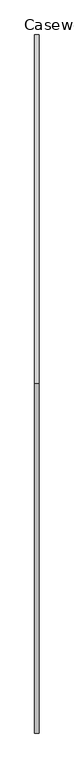
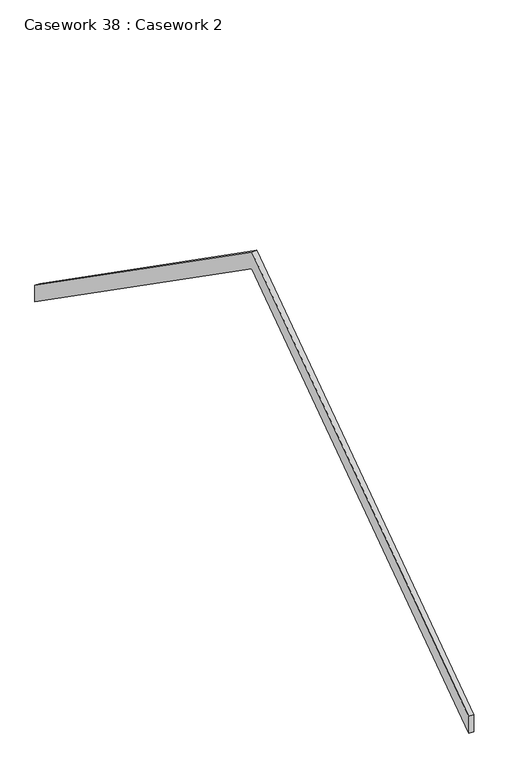
"""IFC4 building model written with IfcOpenShell, lengths in millimetres: furniture geometry, Casework 38 : Casework 2."""

import ifcopenshell
import ifcopenshell.guid

model = None  # the IFC model being written
_history = None  # IfcOwnerHistory: only IFC2X3 demands one
_inside = {}  # id of a spatial element -> (the spatial element, [elements in it])
_under = {}  # id of a project, library or spatial element -> (it, [spatial elements below it])
_declared = {}  # id of a project -> (the project, [libraries it declares])
_typed = {}  # id of a type object -> (the type object, [elements of that type])
_made_of = {}  # id of a material, layer set ... -> (it, [elements and type objects made of it])


def new_model(schema):
    """Start an empty IFC model of exactly this schema.

    Asked for "IFC4X3", IfcOpenShell would pick the latest addendum, in which some entities
    have other attributes; the version numbers below select the first issue.
    IFC2X3 requires an IfcOwnerHistory on every rooted entity: one is made here for all.
    """
    global model, _history
    if schema == "IFC4X3":
        model = ifcopenshell.file(schema_version=(4, 3, 0, 0))
    else:
        model = ifcopenshell.file(schema=schema)
    _inside.clear()
    _under.clear()
    _declared.clear()
    _typed.clear()
    _made_of.clear()
    _history = None
    if model.schema == "IFC2X3":
        org = make("IfcOrganization", Name="unknown")
        user = make(
            "IfcPersonAndOrganization",
            ThePerson=make("IfcPerson", FamilyName="unknown"),
            TheOrganization=org,
        )
        app = make(
            "IfcApplication",
            ApplicationDeveloper=org,
            Version="unknown",
            ApplicationFullName="unknown",
            ApplicationIdentifier="unknown",
        )
        _history = make(
            "IfcOwnerHistory",
            OwningUser=user,
            OwningApplication=app,
            ChangeAction="ADDED",
            CreationDate=0,
        )
    return model


def make(cls, **values):
    """One entity of the class cls with the attributes given. An attribute that is None is left unset."""
    return model.create_entity(
        cls, **{name: value for name, value in values.items() if value is not None}
    )


def rooted(cls, **values):
    """An entity with a GlobalId (a new one), such as an element, a storey or a relation."""
    return make(cls, GlobalId=ifcopenshell.guid.new(), OwnerHistory=_history, **values)


def si_unit(unit_type, name, prefix=None):
    """IfcSIUnit, for example si_unit("LENGTHUNIT", "METRE", prefix="MILLI")."""
    return make("IfcSIUnit", UnitType=unit_type, Prefix=prefix, Name=name)


def assignment(units):
    """IfcUnitAssignment: the units of a project."""
    return None if units is None else make("IfcUnitAssignment", Units=units)


def point(xyz):
    """IfcCartesianPoint."""
    return None if xyz is None else make("IfcCartesianPoint", Coordinates=xyz)


def direction(xyz):
    """IfcDirection."""
    return None if xyz is None else make("IfcDirection", DirectionRatios=xyz)


def frame(location, z_axis=None, x_axis=None):
    """IfcAxis2Placement3D, a coordinate frame: its origin and axes. An axis left out is left unset."""
    return make(
        "IfcAxis2Placement3D",
        Location=point(location),
        Axis=direction(z_axis),
        RefDirection=direction(x_axis),
    )


def origin():
    """The frame at (0, 0, 0) with its axes left unset."""
    return frame((0.0, 0.0, 0.0))


def place(relative_to, where):
    """IfcLocalPlacement: puts the frame where relative to a parent placement (None: the world)."""
    return make(
        "IfcLocalPlacement", PlacementRelTo=relative_to, RelativePlacement=where
    )


def context(
    kind, dimensions, precision=None, world=None, true_north=None, identifier=None
):
    """IfcGeometricRepresentationContext, for example the 3D "Model" context."""
    return make(
        "IfcGeometricRepresentationContext",
        ContextIdentifier=identifier,
        ContextType=kind,
        CoordinateSpaceDimension=dimensions,
        Precision=precision,
        WorldCoordinateSystem=world,
        TrueNorth=true_north,
    )


def project(units=None, contexts=None):
    """IfcProject with its units and contexts."""
    return rooted(
        "IfcProject",
        Name="project",
        RepresentationContexts=contexts,
        UnitsInContext=assignment(units),
    )


def spatial(cls, under=None, at=None, **own):
    """A site, building, storey or space (cls), placed at a placement, below another one or the project."""
    s = rooted(cls, ObjectPlacement=at, **own)
    if under is not None:
        _under.setdefault(under.id(), (under, []))[1].append(s)
    return s


def polyline(points):
    """IfcPolyline through the points."""
    return make("IfcPolyline", Points=[point(p) for p in points])


def outline(outer, holes=None, kind="AREA"):
    """IfcArbitraryClosedProfileDef: a profile drawn as a closed curve; with holes, ...WithVoids."""
    if holes is None:
        return make("IfcArbitraryClosedProfileDef", ProfileType=kind, OuterCurve=outer)
    return make(
        "IfcArbitraryProfileDefWithVoids",
        ProfileType=kind,
        OuterCurve=outer,
        InnerCurves=holes,
    )


def extrude(swept, where, along, depth):
    """IfcExtrudedAreaSolid: the profile swept, set in the frame where, extruded along a direction by depth."""
    return make(
        "IfcExtrudedAreaSolid",
        SweptArea=swept,
        Position=where,
        ExtrudedDirection=direction(along),
        Depth=depth,
    )


def shape(context_of_items, identifier, shape_type, items):
    """IfcShapeRepresentation: the items that make up one representation, for example the "Body"."""
    return make(
        "IfcShapeRepresentation",
        ContextOfItems=context_of_items,
        RepresentationIdentifier=identifier,
        RepresentationType=shape_type,
        Items=items,
    )


def source(mapping_origin, context_of_items, identifier, shape_type, items):
    """IfcRepresentationMap: a shape defined once, which mapped items show again and again."""
    return make(
        "IfcRepresentationMap",
        MappingOrigin=mapping_origin,
        MappedRepresentation=shape(context_of_items, identifier, shape_type, items),
    )


def transform(
    local_origin,
    x_axis=None,
    y_axis=None,
    z_axis=None,
    scale=None,
    scale2=None,
    scale3=None,
    uniform=True,
):
    """IfcCartesianTransformationOperator3D, or its non-uniform kind. x_axis, y_axis, z_axis: its Axis1, 2, 3."""
    if uniform:
        return make(
            "IfcCartesianTransformationOperator3D",
            Axis1=direction(x_axis),
            Axis2=direction(y_axis),
            LocalOrigin=point(local_origin),
            Scale=scale,
            Axis3=direction(z_axis),
        )
    return make(
        "IfcCartesianTransformationOperator3DnonUniform",
        Axis1=direction(x_axis),
        Axis2=direction(y_axis),
        LocalOrigin=point(local_origin),
        Scale=scale,
        Axis3=direction(z_axis),
        Scale2=scale2,
        Scale3=scale3,
    )


def mapped(mapping_source, mapping_target):
    """IfcMappedItem: shows the shape of a source again, moved by a transform."""
    return make(
        "IfcMappedItem", MappingSource=mapping_source, MappingTarget=mapping_target
    )


def made_of(thing, what):
    """Note that an element or type object is made of a material, layer set ...; save() writes the relation."""
    if what is not None:
        _made_of.setdefault(what.id(), (what, []))[1].append(thing)
    return thing


def element(
    cls,
    number,
    at=None,
    inside=None,
    cuts=None,
    type_object=None,
    material=None,
    context=None,
    identifier="Body",
    shape_type=None,
    held_by="IfcProductDefinitionShape",
    body=None,
    shapes=None,
    **own,
):
    """One element of the class cls, such as IfcWall. Its Tag is "e" and its number.

    at: its placement. inside: the storey or other place that contains it. cuts: it is an
    opening in that element (IfcRelVoidsElement). A single representation is given by context,
    identifier, shape_type and body (its items); several are given by shapes. held_by: the class
    of the entity that holds the representations. save() writes the other relations.
    """
    e = rooted(cls, Tag="e%d" % number, ObjectPlacement=at, **own)
    if body is not None:
        shapes = [shape(context, identifier, shape_type, body)]
    if shapes is not None:
        e.Representation = make(held_by, Representations=shapes)
    if inside is not None:
        _inside.setdefault(inside.id(), (inside, []))[1].append(e)
    if cuts is not None:
        rooted(
            "IfcRelVoidsElement", RelatingBuildingElement=cuts, RelatedOpeningElement=e
        )
    if type_object is not None:
        _typed.setdefault(type_object.id(), (type_object, []))[1].append(e)
    return made_of(e, material)


def aggregate(whole, parts):
    """IfcRelAggregates: a whole, such as a stair, and the parts it consists of."""
    return rooted("IfcRelAggregates", RelatingObject=whole, RelatedObjects=parts)


def save(model, path):
    """Write the relations noted so far, then the file.

    IfcRelAggregates (storeys below a building ...), IfcRelContainedInSpatialStructure (elements
    in a storey), IfcRelDefinesByType, IfcRelAssociatesMaterial and IfcRelDeclares: one each for
    every whole, place, type object, material and project.
    """
    for whole, parts in _under.values():
        aggregate(whole, parts)
    for where, things in _inside.values():
        rooted(
            "IfcRelContainedInSpatialStructure",
            RelatedElements=things,
            RelatingStructure=where,
        )
    for kind, things in _typed.values():
        rooted("IfcRelDefinesByType", RelatedObjects=things, RelatingType=kind)
    for what, things in _made_of.values():
        rooted("IfcRelAssociatesMaterial", RelatedObjects=things, RelatingMaterial=what)
    for by, libraries in _declared.values():
        rooted("IfcRelDeclares", RelatingContext=by, RelatedDefinitions=libraries)
    model.write(path)


def casework_38_casework_2_ce946605(model_context):
    return source(origin(), model_context, "Body", "SweptSolid", [
        extrude(outline(polyline([(3152.8649316, 7870.0030963), (7073.1149316, 5125.0144946), (7073.1149316, 4941.8983063), (3152.8649316, 7686.8869079), (-767.3850684, 4941.8983063), (-767.3850684, 5125.0144946), (3152.8649316, 7870.0030963)])), frame((508.4752619, 0.0, 0.0), z_axis=(1.0, 0.0, 0.0), x_axis=(0.0, 1.0, 0.0)), (0.0, 0.0, 1.0), 49.6351915),
    ])


if __name__ == "__main__":
    model = new_model("IFC4")
    model_context = context("Model", 3, world=origin())
    ifc_project = project(units=[si_unit("LENGTHUNIT", "METRE", prefix="MILLI")], contexts=[model_context])
    site = spatial("IfcSite", under=ifc_project)
    building = spatial("IfcBuilding", under=site)
    placement = place(None, origin())
    casework_38_casework_2_shape = casework_38_casework_2_ce946605(model_context)
    element("IfcFurniture", 1, ObjectType="Casework 38 : Casework 2", at=placement, inside=building, context=model_context, shape_type="MappedRepresentation", body=[
        mapped(casework_38_casework_2_shape, transform((0.0, 0.0, 0.0), x_axis=(1.0, 0.0, 0.0), y_axis=(0.0, 1.0, 0.0), z_axis=(0.0, 0.0, 1.0))),
    ])
    save(model, "model.ifc")

# Revit data of these elements
# Project information
#   Document_Suitability_Code = "A1"
#   Document_Suitability_Description = "Coordination"
#   Project Status = "Project Status"
#   Client Name = "Revit Project"
#   Project Address = "Enter address here"
#   Project Name = "Two Storey House"
#   Project Number = "RARC01"
